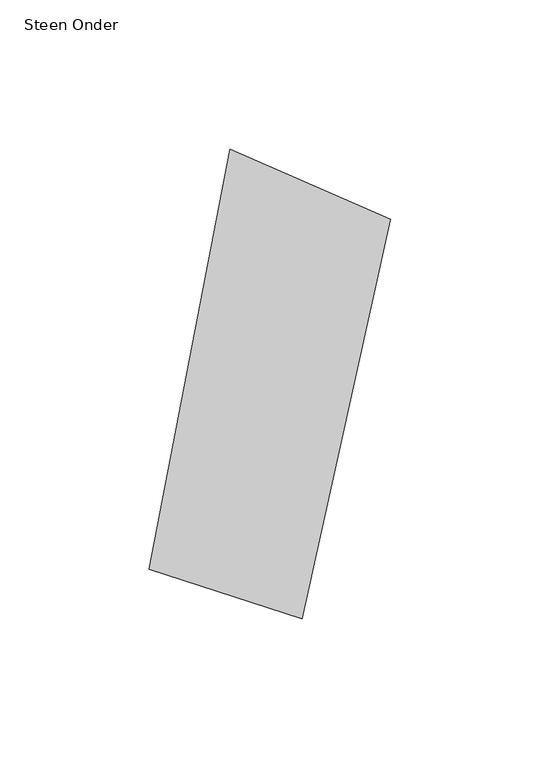
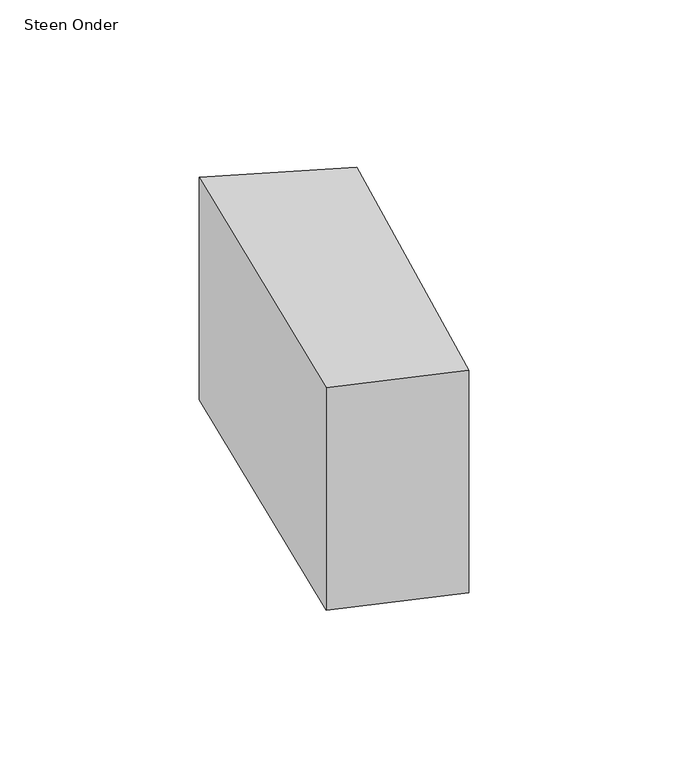
"""IFC4 building model written with IfcOpenShell, lengths in millimetres: proxy geometry, 00_GMA_steen_versie_4 : Steen Onder."""

from ifc_helpers import new_model, si_unit, origin, origin_with_axes, place, context, project, spatial, polyline, outline, extrude, source, transform, mapped, element, save


def steen_onder_d4e6cb58(model_context):
    return source(origin(), model_context, "Body", "SweptSolid", [
        extrude(outline(polyline([(115.1820327, 134.9098002), (85.6120438, 1.2581852), (34.4789915, 17.7778754), (61.585451, 158.2151578), (115.1820327, 134.9098002)])), origin_with_axes(), (0.0, 0.0, 1.0), 100.0),
    ])


if __name__ == "__main__":
    model = new_model("IFC4")
    model_context = context("Model", 3, world=origin())
    ifc_project = project(units=[si_unit("LENGTHUNIT", "METRE", prefix="MILLI")], contexts=[model_context])
    site = spatial("IfcSite", under=ifc_project)
    building = spatial("IfcBuilding", under=site)
    placement = place(None, origin())
    steen_onder_shape = steen_onder_d4e6cb58(model_context)
    element("IfcBuildingElementProxy", 1, Name="00_GMA_steen_versie_4 : Steen Onder", ObjectType="00_GMA_steen_versie_4 : Steen Onder", at=placement, inside=building, context=model_context, shape_type="MappedRepresentation", body=[
        mapped(steen_onder_shape, transform((0.0, 0.0, 0.0), x_axis=(1.0, 0.0, 0.0), y_axis=(0.0, 1.0, 0.0), z_axis=(0.0, 0.0, 1.0))),
    ])
    save(model, "model.ifc")

# Revit data of these elements
# Type "00_GMA_steen_versie_4 : Steen Onder"
#   StootVoegHalfBoven [instance default] = 5 mm
#   StootVoegHalf [instance default] = 5 mm
#   StootVoegBreedteOnder = 10 mm
#   StootVoegBreedteBoven = 10 mm
#   Steendikte = 100 mm
#   LintVoegOnderHalf = 0 mm
#   LintVoegOnder = 0 mm
#   LintVoegBovenHalf = 5 mm
#   LintVoegBoven = 10 mm
#   materiaal = none
#   MateriaalVoeg = none
#   Default Elevation = 0
